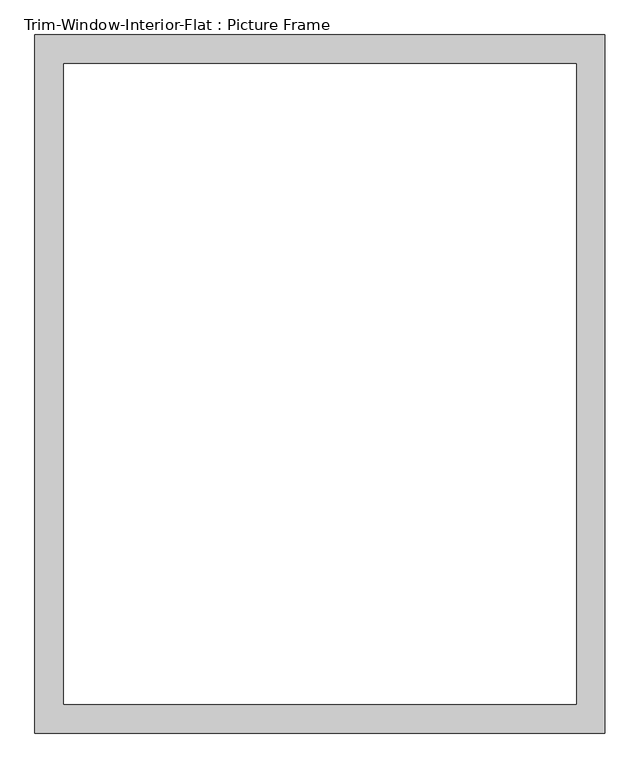
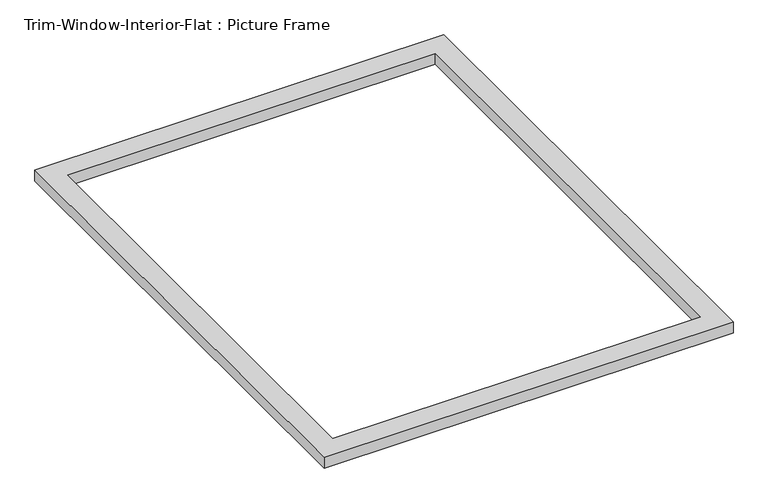
"""IFC4 building model written with IfcOpenShell, lengths in millimetres: proxy geometry, Trim-Window-Interior-Flat : Picture Frame."""

import ifcopenshell
import ifcopenshell.guid

model = None  # the IFC model being written
_history = None  # IfcOwnerHistory: only IFC2X3 demands one
_inside = {}  # id of a spatial element -> (the spatial element, [elements in it])
_under = {}  # id of a project, library or spatial element -> (it, [spatial elements below it])
_declared = {}  # id of a project -> (the project, [libraries it declares])
_typed = {}  # id of a type object -> (the type object, [elements of that type])
_made_of = {}  # id of a material, layer set ... -> (it, [elements and type objects made of it])


def new_model(schema):
    """Start an empty IFC model of exactly this schema.

    Asked for "IFC4X3", IfcOpenShell would pick the latest addendum, in which some entities
    have other attributes; the version numbers below select the first issue.
    IFC2X3 requires an IfcOwnerHistory on every rooted entity: one is made here for all.
    """
    global model, _history
    if schema == "IFC4X3":
        model = ifcopenshell.file(schema_version=(4, 3, 0, 0))
    else:
        model = ifcopenshell.file(schema=schema)
    _inside.clear()
    _under.clear()
    _declared.clear()
    _typed.clear()
    _made_of.clear()
    _history = None
    if model.schema == "IFC2X3":
        org = make("IfcOrganization", Name="unknown")
        user = make(
            "IfcPersonAndOrganization",
            ThePerson=make("IfcPerson", FamilyName="unknown"),
            TheOrganization=org,
        )
        app = make(
            "IfcApplication",
            ApplicationDeveloper=org,
            Version="unknown",
            ApplicationFullName="unknown",
            ApplicationIdentifier="unknown",
        )
        _history = make(
            "IfcOwnerHistory",
            OwningUser=user,
            OwningApplication=app,
            ChangeAction="ADDED",
            CreationDate=0,
        )
    return model


def make(cls, **values):
    """One entity of the class cls with the attributes given. An attribute that is None is left unset."""
    return model.create_entity(
        cls, **{name: value for name, value in values.items() if value is not None}
    )


def rooted(cls, **values):
    """An entity with a GlobalId (a new one), such as an element, a storey or a relation."""
    return make(cls, GlobalId=ifcopenshell.guid.new(), OwnerHistory=_history, **values)


def si_unit(unit_type, name, prefix=None):
    """IfcSIUnit, for example si_unit("LENGTHUNIT", "METRE", prefix="MILLI")."""
    return make("IfcSIUnit", UnitType=unit_type, Prefix=prefix, Name=name)


def assignment(units):
    """IfcUnitAssignment: the units of a project."""
    return None if units is None else make("IfcUnitAssignment", Units=units)


def point(xyz):
    """IfcCartesianPoint."""
    return None if xyz is None else make("IfcCartesianPoint", Coordinates=xyz)


def direction(xyz):
    """IfcDirection."""
    return None if xyz is None else make("IfcDirection", DirectionRatios=xyz)


def frame(location, z_axis=None, x_axis=None):
    """IfcAxis2Placement3D, a coordinate frame: its origin and axes. An axis left out is left unset."""
    return make(
        "IfcAxis2Placement3D",
        Location=point(location),
        Axis=direction(z_axis),
        RefDirection=direction(x_axis),
    )


def origin():
    """The frame at (0, 0, 0) with its axes left unset."""
    return frame((0.0, 0.0, 0.0))


def origin_with_axes():
    """The frame at (0, 0, 0) with the z axis (0, 0, 1) and the x axis (1, 0, 0) written out."""
    return frame((0.0, 0.0, 0.0), z_axis=(0.0, 0.0, 1.0), x_axis=(1.0, 0.0, 0.0))


def place(relative_to, where):
    """IfcLocalPlacement: puts the frame where relative to a parent placement (None: the world)."""
    return make(
        "IfcLocalPlacement", PlacementRelTo=relative_to, RelativePlacement=where
    )


def context(
    kind, dimensions, precision=None, world=None, true_north=None, identifier=None
):
    """IfcGeometricRepresentationContext, for example the 3D "Model" context."""
    return make(
        "IfcGeometricRepresentationContext",
        ContextIdentifier=identifier,
        ContextType=kind,
        CoordinateSpaceDimension=dimensions,
        Precision=precision,
        WorldCoordinateSystem=world,
        TrueNorth=true_north,
    )


def project(units=None, contexts=None):
    """IfcProject with its units and contexts."""
    return rooted(
        "IfcProject",
        Name="project",
        RepresentationContexts=contexts,
        UnitsInContext=assignment(units),
    )


def spatial(cls, under=None, at=None, **own):
    """A site, building, storey or space (cls), placed at a placement, below another one or the project."""
    s = rooted(cls, ObjectPlacement=at, **own)
    if under is not None:
        _under.setdefault(under.id(), (under, []))[1].append(s)
    return s


def polyline(points):
    """IfcPolyline through the points."""
    return make("IfcPolyline", Points=[point(p) for p in points])


def outline(outer, holes=None, kind="AREA"):
    """IfcArbitraryClosedProfileDef: a profile drawn as a closed curve; with holes, ...WithVoids."""
    if holes is None:
        return make("IfcArbitraryClosedProfileDef", ProfileType=kind, OuterCurve=outer)
    return make(
        "IfcArbitraryProfileDefWithVoids",
        ProfileType=kind,
        OuterCurve=outer,
        InnerCurves=holes,
    )


def extrude(swept, where, along, depth):
    """IfcExtrudedAreaSolid: the profile swept, set in the frame where, extruded along a direction by depth."""
    return make(
        "IfcExtrudedAreaSolid",
        SweptArea=swept,
        Position=where,
        ExtrudedDirection=direction(along),
        Depth=depth,
    )


def shape(context_of_items, identifier, shape_type, items):
    """IfcShapeRepresentation: the items that make up one representation, for example the "Body"."""
    return make(
        "IfcShapeRepresentation",
        ContextOfItems=context_of_items,
        RepresentationIdentifier=identifier,
        RepresentationType=shape_type,
        Items=items,
    )


def source(mapping_origin, context_of_items, identifier, shape_type, items):
    """IfcRepresentationMap: a shape defined once, which mapped items show again and again."""
    return make(
        "IfcRepresentationMap",
        MappingOrigin=mapping_origin,
        MappedRepresentation=shape(context_of_items, identifier, shape_type, items),
    )


def transform(
    local_origin,
    x_axis=None,
    y_axis=None,
    z_axis=None,
    scale=None,
    scale2=None,
    scale3=None,
    uniform=True,
):
    """IfcCartesianTransformationOperator3D, or its non-uniform kind. x_axis, y_axis, z_axis: its Axis1, 2, 3."""
    if uniform:
        return make(
            "IfcCartesianTransformationOperator3D",
            Axis1=direction(x_axis),
            Axis2=direction(y_axis),
            LocalOrigin=point(local_origin),
            Scale=scale,
            Axis3=direction(z_axis),
        )
    return make(
        "IfcCartesianTransformationOperator3DnonUniform",
        Axis1=direction(x_axis),
        Axis2=direction(y_axis),
        LocalOrigin=point(local_origin),
        Scale=scale,
        Axis3=direction(z_axis),
        Scale2=scale2,
        Scale3=scale3,
    )


def mapped(mapping_source, mapping_target):
    """IfcMappedItem: shows the shape of a source again, moved by a transform."""
    return make(
        "IfcMappedItem", MappingSource=mapping_source, MappingTarget=mapping_target
    )


def made_of(thing, what):
    """Note that an element or type object is made of a material, layer set ...; save() writes the relation."""
    if what is not None:
        _made_of.setdefault(what.id(), (what, []))[1].append(thing)
    return thing


def element(
    cls,
    number,
    at=None,
    inside=None,
    cuts=None,
    type_object=None,
    material=None,
    context=None,
    identifier="Body",
    shape_type=None,
    held_by="IfcProductDefinitionShape",
    body=None,
    shapes=None,
    **own,
):
    """One element of the class cls, such as IfcWall. Its Tag is "e" and its number.

    at: its placement. inside: the storey or other place that contains it. cuts: it is an
    opening in that element (IfcRelVoidsElement). A single representation is given by context,
    identifier, shape_type and body (its items); several are given by shapes. held_by: the class
    of the entity that holds the representations. save() writes the other relations.
    """
    e = rooted(cls, Tag="e%d" % number, ObjectPlacement=at, **own)
    if body is not None:
        shapes = [shape(context, identifier, shape_type, body)]
    if shapes is not None:
        e.Representation = make(held_by, Representations=shapes)
    if inside is not None:
        _inside.setdefault(inside.id(), (inside, []))[1].append(e)
    if cuts is not None:
        rooted(
            "IfcRelVoidsElement", RelatingBuildingElement=cuts, RelatedOpeningElement=e
        )
    if type_object is not None:
        _typed.setdefault(type_object.id(), (type_object, []))[1].append(e)
    return made_of(e, material)


def aggregate(whole, parts):
    """IfcRelAggregates: a whole, such as a stair, and the parts it consists of."""
    return rooted("IfcRelAggregates", RelatingObject=whole, RelatedObjects=parts)


def save(model, path):
    """Write the relations noted so far, then the file.

    IfcRelAggregates (storeys below a building ...), IfcRelContainedInSpatialStructure (elements
    in a storey), IfcRelDefinesByType, IfcRelAssociatesMaterial and IfcRelDeclares: one each for
    every whole, place, type object, material and project.
    """
    for whole, parts in _under.values():
        aggregate(whole, parts)
    for where, things in _inside.values():
        rooted(
            "IfcRelContainedInSpatialStructure",
            RelatedElements=things,
            RelatingStructure=where,
        )
    for kind, things in _typed.values():
        rooted("IfcRelDefinesByType", RelatedObjects=things, RelatingType=kind)
    for what, things in _made_of.values():
        rooted("IfcRelAssociatesMaterial", RelatedObjects=things, RelatingMaterial=what)
    for by, libraries in _declared.values():
        rooted("IfcRelDeclares", RelatingContext=by, RelatedDefinitions=libraries)
    model.write(path)


def trim_window_interior_flat_picture_frame_b488ca0e(model_context):
    return source(origin(), model_context, "Body", "SweptSolid", [
        extrude(outline(polyline([(565.15, 44.45), (565.15, -1339.85), (-565.15, -1339.85), (-565.15, 44.45), (565.15, 44.45)]), holes=[polyline([(508.0, -12.7), (-508.0, -12.7), (-508.0, -1282.7), (508.0, -1282.7), (508.0, -12.7)])]), origin_with_axes(), (0.0, 0.0, 1.0), 31.75),
    ])


if __name__ == "__main__":
    model = new_model("IFC4")
    model_context = context("Model", 3, world=origin())
    ifc_project = project(units=[si_unit("LENGTHUNIT", "METRE", prefix="MILLI")], contexts=[model_context])
    site = spatial("IfcSite", under=ifc_project)
    building = spatial("IfcBuilding", under=site)
    placement = place(None, origin())
    trim_window_interior_flat_picture_frame_shape = trim_window_interior_flat_picture_frame_b488ca0e(model_context)
    element("IfcBuildingElementProxy", 1, Name="Trim-Window-Interior-Flat : Picture Frame", ObjectType="Trim-Window-Interior-Flat : Picture Frame", at=placement, inside=building, context=model_context, shape_type="MappedRepresentation", body=[
        mapped(trim_window_interior_flat_picture_frame_shape, transform((0.0, 0.0, 0.0), x_axis=(1.0, 0.0, 0.0), y_axis=(0.0, 1.0, 0.0), z_axis=(0.0, 0.0, 1.0))),
    ])
    save(model, "model.ifc")

# Revit data of these elements
# Type "Trim-Window-Interior-Flat : Picture Frame"
#   Trim Thickness_Picture Frame = 0' - 1 1/4"
#   Trim Width = 0' - 2 1/4"
#   Trim Thickness_with Sill = 0' - 0 3/4"
#   Sill Thickness = 0' - 1 1/4"
#   Opening Width [instance default] = 2' - 0"
#   Opening Height [instance default] = 3' - 0"
#   Default Elevation = 4' - 0"
#   Sill = no
#   Picture Frame = yes
#   Trim Material [instance default] = none
# Element 1 (IfcBuildingElementProxy, "Trim-Window-Interior-Flat : Picture Frame")
#   Opening Width = 3' - 5"
#   Opening Height = 4' - 3"
#   Trim Material = Wood - Stained
#   Materials on its faces: "Wood - Stained"
# Materials
#   "Wood - Stained": class "Wood", colour RGB 224 178 126, transparency 0, Cost = 0
